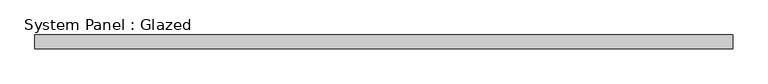
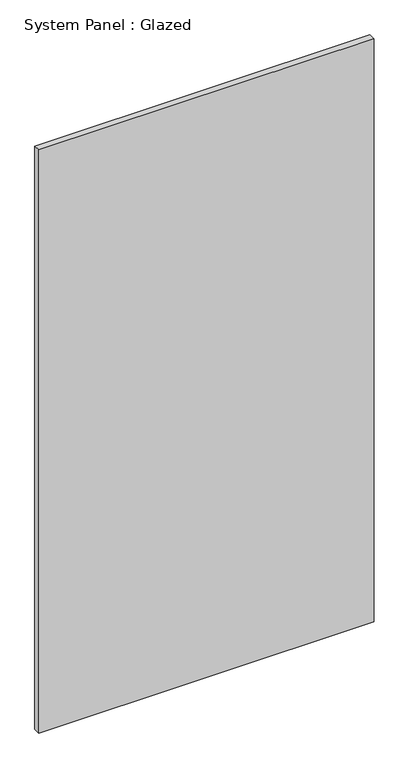
"""IFC4 building model written with IfcOpenShell, lengths in millimetres: plate geometry, System Panel : Glazed."""

import ifcopenshell
import ifcopenshell.guid

model = None  # the IFC model being written
_history = None  # IfcOwnerHistory: only IFC2X3 demands one
_inside = {}  # id of a spatial element -> (the spatial element, [elements in it])
_under = {}  # id of a project, library or spatial element -> (it, [spatial elements below it])
_declared = {}  # id of a project -> (the project, [libraries it declares])
_typed = {}  # id of a type object -> (the type object, [elements of that type])
_made_of = {}  # id of a material, layer set ... -> (it, [elements and type objects made of it])


def new_model(schema):
    """Start an empty IFC model of exactly this schema.

    Asked for "IFC4X3", IfcOpenShell would pick the latest addendum, in which some entities
    have other attributes; the version numbers below select the first issue.
    IFC2X3 requires an IfcOwnerHistory on every rooted entity: one is made here for all.
    """
    global model, _history
    if schema == "IFC4X3":
        model = ifcopenshell.file(schema_version=(4, 3, 0, 0))
    else:
        model = ifcopenshell.file(schema=schema)
    _inside.clear()
    _under.clear()
    _declared.clear()
    _typed.clear()
    _made_of.clear()
    _history = None
    if model.schema == "IFC2X3":
        org = make("IfcOrganization", Name="unknown")
        user = make(
            "IfcPersonAndOrganization",
            ThePerson=make("IfcPerson", FamilyName="unknown"),
            TheOrganization=org,
        )
        app = make(
            "IfcApplication",
            ApplicationDeveloper=org,
            Version="unknown",
            ApplicationFullName="unknown",
            ApplicationIdentifier="unknown",
        )
        _history = make(
            "IfcOwnerHistory",
            OwningUser=user,
            OwningApplication=app,
            ChangeAction="ADDED",
            CreationDate=0,
        )
    return model


def make(cls, **values):
    """One entity of the class cls with the attributes given. An attribute that is None is left unset."""
    return model.create_entity(
        cls, **{name: value for name, value in values.items() if value is not None}
    )


def rooted(cls, **values):
    """An entity with a GlobalId (a new one), such as an element, a storey or a relation."""
    return make(cls, GlobalId=ifcopenshell.guid.new(), OwnerHistory=_history, **values)


def si_unit(unit_type, name, prefix=None):
    """IfcSIUnit, for example si_unit("LENGTHUNIT", "METRE", prefix="MILLI")."""
    return make("IfcSIUnit", UnitType=unit_type, Prefix=prefix, Name=name)


def assignment(units):
    """IfcUnitAssignment: the units of a project."""
    return None if units is None else make("IfcUnitAssignment", Units=units)


def point(xyz):
    """IfcCartesianPoint."""
    return None if xyz is None else make("IfcCartesianPoint", Coordinates=xyz)


def direction(xyz):
    """IfcDirection."""
    return None if xyz is None else make("IfcDirection", DirectionRatios=xyz)


def frame(location, z_axis=None, x_axis=None):
    """IfcAxis2Placement3D, a coordinate frame: its origin and axes. An axis left out is left unset."""
    return make(
        "IfcAxis2Placement3D",
        Location=point(location),
        Axis=direction(z_axis),
        RefDirection=direction(x_axis),
    )


def origin():
    """The frame at (0, 0, 0) with its axes left unset."""
    return frame((0.0, 0.0, 0.0))


def origin_with_axes():
    """The frame at (0, 0, 0) with the z axis (0, 0, 1) and the x axis (1, 0, 0) written out."""
    return frame((0.0, 0.0, 0.0), z_axis=(0.0, 0.0, 1.0), x_axis=(1.0, 0.0, 0.0))


def place(relative_to, where):
    """IfcLocalPlacement: puts the frame where relative to a parent placement (None: the world)."""
    return make(
        "IfcLocalPlacement", PlacementRelTo=relative_to, RelativePlacement=where
    )


def context(
    kind, dimensions, precision=None, world=None, true_north=None, identifier=None
):
    """IfcGeometricRepresentationContext, for example the 3D "Model" context."""
    return make(
        "IfcGeometricRepresentationContext",
        ContextIdentifier=identifier,
        ContextType=kind,
        CoordinateSpaceDimension=dimensions,
        Precision=precision,
        WorldCoordinateSystem=world,
        TrueNorth=true_north,
    )


def project(units=None, contexts=None):
    """IfcProject with its units and contexts."""
    return rooted(
        "IfcProject",
        Name="project",
        RepresentationContexts=contexts,
        UnitsInContext=assignment(units),
    )


def spatial(cls, under=None, at=None, **own):
    """A site, building, storey or space (cls), placed at a placement, below another one or the project."""
    s = rooted(cls, ObjectPlacement=at, **own)
    if under is not None:
        _under.setdefault(under.id(), (under, []))[1].append(s)
    return s


def polyline(points):
    """IfcPolyline through the points."""
    return make("IfcPolyline", Points=[point(p) for p in points])


def outline(outer, holes=None, kind="AREA"):
    """IfcArbitraryClosedProfileDef: a profile drawn as a closed curve; with holes, ...WithVoids."""
    if holes is None:
        return make("IfcArbitraryClosedProfileDef", ProfileType=kind, OuterCurve=outer)
    return make(
        "IfcArbitraryProfileDefWithVoids",
        ProfileType=kind,
        OuterCurve=outer,
        InnerCurves=holes,
    )


def extrude(swept, where, along, depth):
    """IfcExtrudedAreaSolid: the profile swept, set in the frame where, extruded along a direction by depth."""
    return make(
        "IfcExtrudedAreaSolid",
        SweptArea=swept,
        Position=where,
        ExtrudedDirection=direction(along),
        Depth=depth,
    )


def shape(context_of_items, identifier, shape_type, items):
    """IfcShapeRepresentation: the items that make up one representation, for example the "Body"."""
    return make(
        "IfcShapeRepresentation",
        ContextOfItems=context_of_items,
        RepresentationIdentifier=identifier,
        RepresentationType=shape_type,
        Items=items,
    )


def source(mapping_origin, context_of_items, identifier, shape_type, items):
    """IfcRepresentationMap: a shape defined once, which mapped items show again and again."""
    return make(
        "IfcRepresentationMap",
        MappingOrigin=mapping_origin,
        MappedRepresentation=shape(context_of_items, identifier, shape_type, items),
    )


def transform(
    local_origin,
    x_axis=None,
    y_axis=None,
    z_axis=None,
    scale=None,
    scale2=None,
    scale3=None,
    uniform=True,
):
    """IfcCartesianTransformationOperator3D, or its non-uniform kind. x_axis, y_axis, z_axis: its Axis1, 2, 3."""
    if uniform:
        return make(
            "IfcCartesianTransformationOperator3D",
            Axis1=direction(x_axis),
            Axis2=direction(y_axis),
            LocalOrigin=point(local_origin),
            Scale=scale,
            Axis3=direction(z_axis),
        )
    return make(
        "IfcCartesianTransformationOperator3DnonUniform",
        Axis1=direction(x_axis),
        Axis2=direction(y_axis),
        LocalOrigin=point(local_origin),
        Scale=scale,
        Axis3=direction(z_axis),
        Scale2=scale2,
        Scale3=scale3,
    )


def mapped(mapping_source, mapping_target):
    """IfcMappedItem: shows the shape of a source again, moved by a transform."""
    return make(
        "IfcMappedItem", MappingSource=mapping_source, MappingTarget=mapping_target
    )


def made_of(thing, what):
    """Note that an element or type object is made of a material, layer set ...; save() writes the relation."""
    if what is not None:
        _made_of.setdefault(what.id(), (what, []))[1].append(thing)
    return thing


def element(
    cls,
    number,
    at=None,
    inside=None,
    cuts=None,
    type_object=None,
    material=None,
    context=None,
    identifier="Body",
    shape_type=None,
    held_by="IfcProductDefinitionShape",
    body=None,
    shapes=None,
    **own,
):
    """One element of the class cls, such as IfcWall. Its Tag is "e" and its number.

    at: its placement. inside: the storey or other place that contains it. cuts: it is an
    opening in that element (IfcRelVoidsElement). A single representation is given by context,
    identifier, shape_type and body (its items); several are given by shapes. held_by: the class
    of the entity that holds the representations. save() writes the other relations.
    """
    e = rooted(cls, Tag="e%d" % number, ObjectPlacement=at, **own)
    if body is not None:
        shapes = [shape(context, identifier, shape_type, body)]
    if shapes is not None:
        e.Representation = make(held_by, Representations=shapes)
    if inside is not None:
        _inside.setdefault(inside.id(), (inside, []))[1].append(e)
    if cuts is not None:
        rooted(
            "IfcRelVoidsElement", RelatingBuildingElement=cuts, RelatedOpeningElement=e
        )
    if type_object is not None:
        _typed.setdefault(type_object.id(), (type_object, []))[1].append(e)
    return made_of(e, material)


def aggregate(whole, parts):
    """IfcRelAggregates: a whole, such as a stair, and the parts it consists of."""
    return rooted("IfcRelAggregates", RelatingObject=whole, RelatedObjects=parts)


def save(model, path):
    """Write the relations noted so far, then the file.

    IfcRelAggregates (storeys below a building ...), IfcRelContainedInSpatialStructure (elements
    in a storey), IfcRelDefinesByType, IfcRelAssociatesMaterial and IfcRelDeclares: one each for
    every whole, place, type object, material and project.
    """
    for whole, parts in _under.values():
        aggregate(whole, parts)
    for where, things in _inside.values():
        rooted(
            "IfcRelContainedInSpatialStructure",
            RelatedElements=things,
            RelatingStructure=where,
        )
    for kind, things in _typed.values():
        rooted("IfcRelDefinesByType", RelatedObjects=things, RelatingType=kind)
    for what, things in _made_of.values():
        rooted("IfcRelAssociatesMaterial", RelatedObjects=things, RelatingMaterial=what)
    for by, libraries in _declared.values():
        rooted("IfcRelDeclares", RelatingContext=by, RelatedDefinitions=libraries)
    model.write(path)


def system_panel_glazed_e4649fa4(model_context):
    return source(origin(), model_context, "Body", "SweptSolid", [
        extrude(outline(polyline([(632.4999999, 24.5), (-632.4999999, 24.5), (-632.4999999, 49.5), (632.4999999, 49.5), (632.4999999, 24.5)])), origin_with_axes(), (0.0, 0.0, 1.0), 2325.0),
    ])


if __name__ == "__main__":
    model = new_model("IFC4")
    model_context = context("Model", 3, world=origin())
    ifc_project = project(units=[si_unit("LENGTHUNIT", "METRE", prefix="MILLI")], contexts=[model_context])
    site = spatial("IfcSite", under=ifc_project)
    building = spatial("IfcBuilding", under=site)
    placement = place(None, origin())
    system_panel_glazed_shape = system_panel_glazed_e4649fa4(model_context)
    element("IfcPlate", 1, ObjectType="System Panel : Glazed", at=placement, inside=building, context=model_context, shape_type="MappedRepresentation", body=[
        mapped(system_panel_glazed_shape, transform((0.0, 0.0, 0.0), x_axis=(1.0, 0.0, 0.0), y_axis=(0.0, 1.0, 0.0), z_axis=(0.0, 0.0, 1.0))),
    ])
    save(model, "model.ifc")

# Revit data of these elements
# Type "System Panel : Glazed"
#   Construction Type Id = "GSP4R"
#   Analytic Construction = "1/8 in Pilkington single glazing"
#   Visual Light Transmittance = 0.9
#   Solar Heat Gain Coefficient = 0.86
#   Heat Transfer Coefficient (U) = 6.7069 W/(m²·K)
#   Define Thermal Properties by = 1
# Element 1 (IfcPlate, "System Panel : Glazed")
#   Materials on its faces: "Glass"
# Materials
#   "Glass": class "Glass", colour RGB 0 128 192, transparency 0.9, Description = "Soda Lime Glass", Cost = 0
